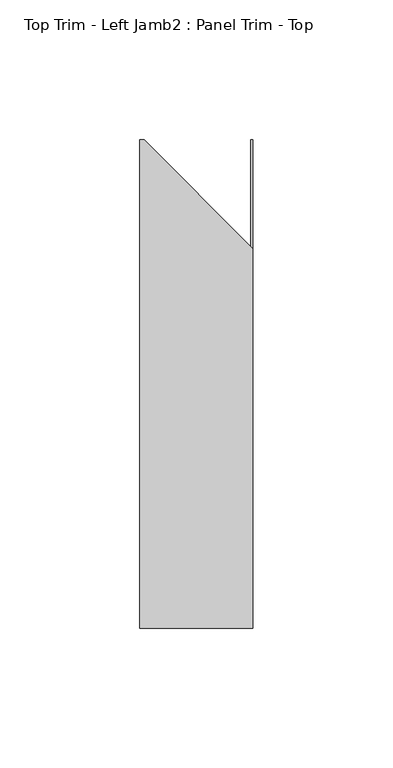
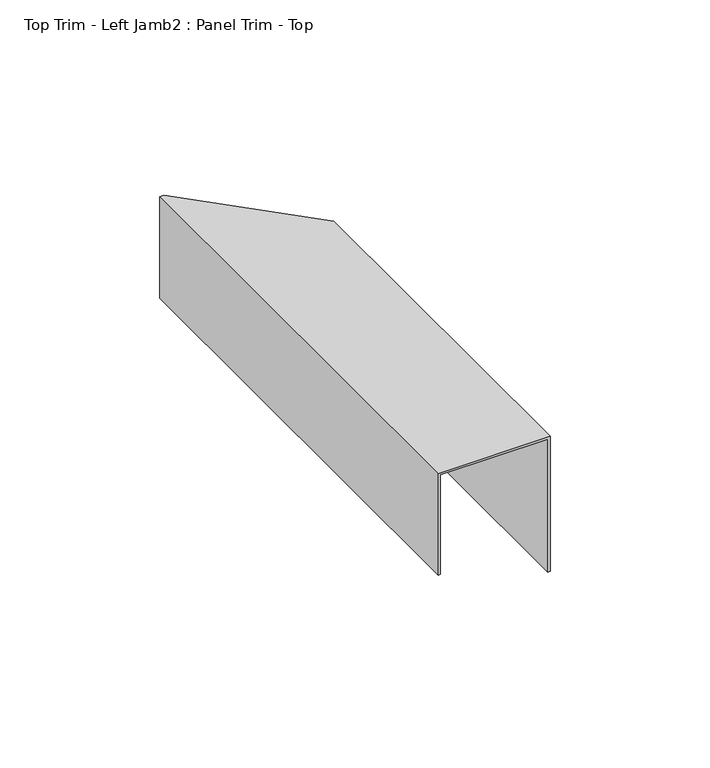
"""IFC4 building model written with IfcOpenShell, lengths in millimetres: proxy geometry, Top Trim - Left Jamb2 : Panel Trim - Top."""

from ifc_helpers import new_model, si_unit, origin, place, context, project, spatial, faceted_brep, source, transform, mapped, element, save


def top_trim_left_jamb2_panel_trim_top_cc1ac03c(model_context):
    return source(origin(), model_context, "Body", "Brep", [
        faceted_brep([(587327.0060739, -531601.1163841, 2439.9875), (587327.0060739, -531601.1163841, 2401.8875), (587326.2186739, -531601.1163841, 2401.8875), (587326.2186739, -531601.1163841, 2440.78125), (587327.7847411, -531601.1163841, 2440.78125), (587327.7847411, -531601.1163841, 2439.9875), (587366.6808739, -531601.1163841, 2389.1875), (587365.8934739, -531601.1163841, 2389.1875), (587365.8934739, -531601.1163841, 2413.0), (587366.6808739, -531601.1163841, 2413.0), (587327.0060739, -531775.7413841, 2439.9875), (587365.8934739, -531775.7413841, 2439.9875), (587365.8934739, -531775.7413841, 2389.1875), (587366.6808739, -531775.7413841, 2389.1875), (587366.6808739, -531775.7413841, 2440.78125), (587326.2186739, -531775.7413841, 2440.78125), (587326.2186739, -531775.7413841, 2401.8875), (587327.0060739, -531775.7413841, 2401.8875), (587366.6808739, -531640.0125169, 2440.78125), (587366.6808739, -531640.0125169, 2413.0), (587365.8934739, -531639.2251169, 2439.9875), (587365.8934739, -531639.2251169, 2413.0)], [[[0, 1, 2, 3, 4, 5]], [[6, 7, 8, 9]], [[10, 11, 12, 13, 14, 15, 16, 17]], [[1, 0, 10, 17]], [[2, 1, 17, 16]], [[3, 2, 16, 15]], [[15, 14, 18, 4, 3]], [[14, 13, 6, 9, 19, 18]], [[7, 6, 13, 12]], [[12, 11, 20, 21, 8, 7]], [[11, 10, 0, 5, 20]], [[21, 19, 9, 8]], [[19, 21, 20, 5, 4, 18]]]),
    ])


if __name__ == "__main__":
    model = new_model("IFC4")
    model_context = context("Model", 3, world=origin())
    ifc_project = project(units=[si_unit("LENGTHUNIT", "METRE", prefix="MILLI")], contexts=[model_context])
    site = spatial("IfcSite", under=ifc_project)
    building = spatial("IfcBuilding", under=site)
    placement = place(None, origin())
    top_trim_left_jamb2_panel_trim_top_shape = top_trim_left_jamb2_panel_trim_top_cc1ac03c(model_context)
    element("IfcBuildingElementProxy", 1, Name="Top Trim - Left Jamb2 : Panel Trim - Top", ObjectType="Top Trim - Left Jamb2 : Panel Trim - Top", at=placement, inside=building, context=model_context, shape_type="MappedRepresentation", body=[
        mapped(top_trim_left_jamb2_panel_trim_top_shape, transform((0.0, 0.0, 0.0), x_axis=(1.0, 0.0, 0.0), y_axis=(0.0, 1.0, 0.0), z_axis=(0.0, 0.0, 1.0))),
    ])
    save(model, "model.ifc")

# Revit data of these elements
# Element 1 (IfcBuildingElementProxy, "Top Trim - Left Jamb2 : Panel Trim - Top")
#   Materials on its faces: "EDGE TRIM BY MTL PANEL MFR."
# Materials
#   "EDGE TRIM BY MTL PANEL MFR.": class "Generic", colour RGB 239 242 240, transparency 0, Cost = 0
